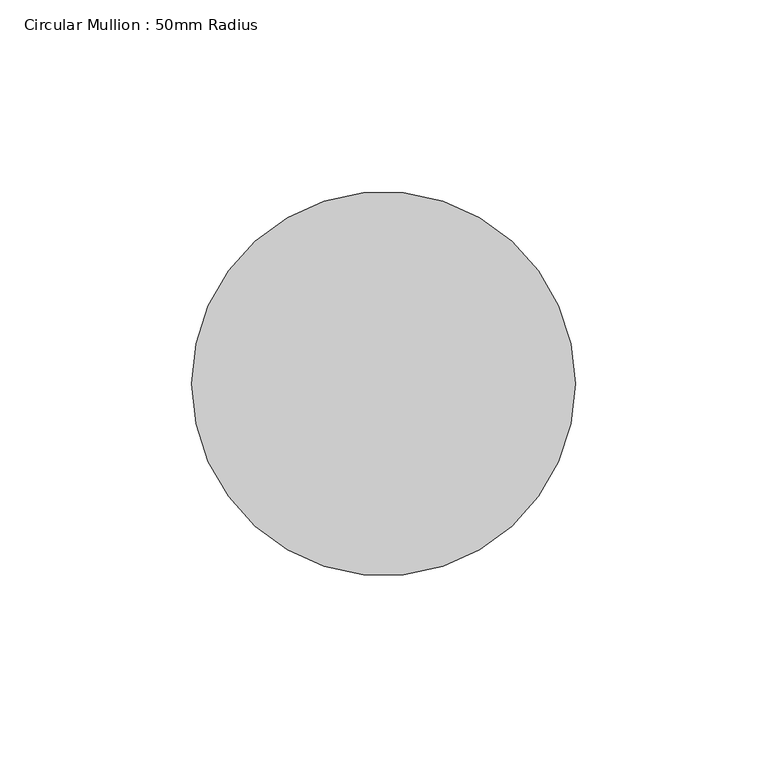
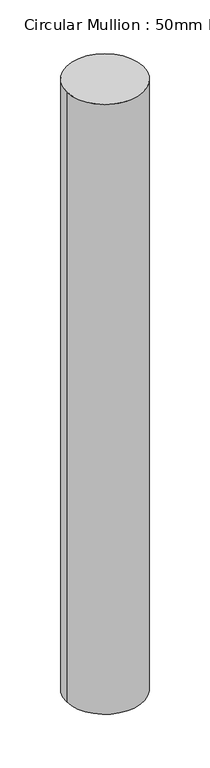
"""IFC4 building model written with IfcOpenShell, lengths in millimetres: member geometry, Circular Mullion : 50mm Radius."""

from ifc_helpers import new_model, si_unit, point, frame, origin, origin_2d, place, context, project, spatial, circle_curve, trimmed, segment, composite_curve, outline, extrude, source, transform, mapped, element, save


def circular_mullion_50mm_radius_52b26596(model_context):
    return source(origin(), model_context, "Body", "SweptSolid", [
        extrude(outline(composite_curve([segment(trimmed(circle_curve(origin_2d(), 50.0), [point((50.0, 0.0))], [point((-50.0, 0.0))], False, "CARTESIAN"), True, "CONTINUOUS"), segment(trimmed(circle_curve(origin_2d(), 50.0), [point((-50.0, 0.0))], [point((50.0, 0.0))], False, "CARTESIAN"), True, "CONTINUOUS")], self_intersect=False)), frame((0.0, 0.0, -839.4364191), z_axis=(0.0, 0.0, 1.0), x_axis=(1.0, 0.0, 0.0)), (0.0, 0.0, 1.0), 839.4364191),
    ])


if __name__ == "__main__":
    model = new_model("IFC4")
    model_context = context("Model", 3, world=origin())
    ifc_project = project(units=[si_unit("LENGTHUNIT", "METRE", prefix="MILLI")], contexts=[model_context])
    site = spatial("IfcSite", under=ifc_project)
    building = spatial("IfcBuilding", under=site)
    placement = place(None, origin())
    circular_mullion_50mm_radius_shape = circular_mullion_50mm_radius_52b26596(model_context)
    element("IfcMember", 1, ObjectType="Circular Mullion : 50mm Radius", at=placement, inside=building, context=model_context, shape_type="MappedRepresentation", body=[
        mapped(circular_mullion_50mm_radius_shape, transform((0.0, 0.0, 0.0), x_axis=(1.0, 0.0, 0.0), y_axis=(0.0, 1.0, 0.0), z_axis=(0.0, 0.0, 1.0))),
    ])
    save(model, "model.ifc")

# Revit data of these elements
# Type "Circular Mullion : 50mm Radius"
#   built-in parameter 1007350 = 0.164042 (stored number, unit not read)
# Element 1 (IfcMember, "Circular Mullion : 50mm Radius")
#   Materials on its faces: "Aluminium"
# Materials
#   "Aluminium": class "Metal", colour RGB 247 247 247, transparency 0, Description = "Aluminium 6061", Cost = 0
